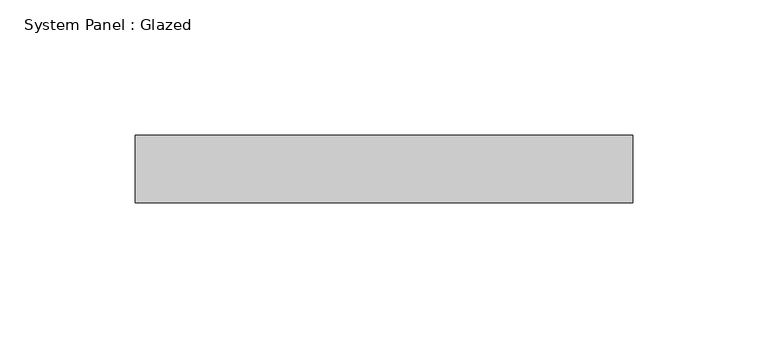
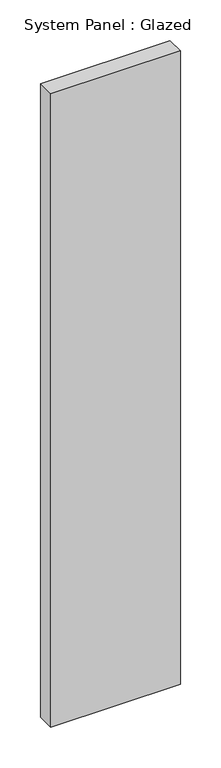
"""IFC4 building model written with IfcOpenShell, lengths in millimetres: plate geometry, System Panel : Glazed."""

import ifcopenshell
import ifcopenshell.guid

model = None  # the IFC model being written
_history = None  # IfcOwnerHistory: only IFC2X3 demands one
_inside = {}  # id of a spatial element -> (the spatial element, [elements in it])
_under = {}  # id of a project, library or spatial element -> (it, [spatial elements below it])
_declared = {}  # id of a project -> (the project, [libraries it declares])
_typed = {}  # id of a type object -> (the type object, [elements of that type])
_made_of = {}  # id of a material, layer set ... -> (it, [elements and type objects made of it])


def new_model(schema):
    """Start an empty IFC model of exactly this schema.

    Asked for "IFC4X3", IfcOpenShell would pick the latest addendum, in which some entities
    have other attributes; the version numbers below select the first issue.
    IFC2X3 requires an IfcOwnerHistory on every rooted entity: one is made here for all.
    """
    global model, _history
    if schema == "IFC4X3":
        model = ifcopenshell.file(schema_version=(4, 3, 0, 0))
    else:
        model = ifcopenshell.file(schema=schema)
    _inside.clear()
    _under.clear()
    _declared.clear()
    _typed.clear()
    _made_of.clear()
    _history = None
    if model.schema == "IFC2X3":
        org = make("IfcOrganization", Name="unknown")
        user = make(
            "IfcPersonAndOrganization",
            ThePerson=make("IfcPerson", FamilyName="unknown"),
            TheOrganization=org,
        )
        app = make(
            "IfcApplication",
            ApplicationDeveloper=org,
            Version="unknown",
            ApplicationFullName="unknown",
            ApplicationIdentifier="unknown",
        )
        _history = make(
            "IfcOwnerHistory",
            OwningUser=user,
            OwningApplication=app,
            ChangeAction="ADDED",
            CreationDate=0,
        )
    return model


def make(cls, **values):
    """One entity of the class cls with the attributes given. An attribute that is None is left unset."""
    return model.create_entity(
        cls, **{name: value for name, value in values.items() if value is not None}
    )


def rooted(cls, **values):
    """An entity with a GlobalId (a new one), such as an element, a storey or a relation."""
    return make(cls, GlobalId=ifcopenshell.guid.new(), OwnerHistory=_history, **values)


def si_unit(unit_type, name, prefix=None):
    """IfcSIUnit, for example si_unit("LENGTHUNIT", "METRE", prefix="MILLI")."""
    return make("IfcSIUnit", UnitType=unit_type, Prefix=prefix, Name=name)


def assignment(units):
    """IfcUnitAssignment: the units of a project."""
    return None if units is None else make("IfcUnitAssignment", Units=units)


def point(xyz):
    """IfcCartesianPoint."""
    return None if xyz is None else make("IfcCartesianPoint", Coordinates=xyz)


def direction(xyz):
    """IfcDirection."""
    return None if xyz is None else make("IfcDirection", DirectionRatios=xyz)


def frame(location, z_axis=None, x_axis=None):
    """IfcAxis2Placement3D, a coordinate frame: its origin and axes. An axis left out is left unset."""
    return make(
        "IfcAxis2Placement3D",
        Location=point(location),
        Axis=direction(z_axis),
        RefDirection=direction(x_axis),
    )


def origin():
    """The frame at (0, 0, 0) with its axes left unset."""
    return frame((0.0, 0.0, 0.0))


def origin_with_axes():
    """The frame at (0, 0, 0) with the z axis (0, 0, 1) and the x axis (1, 0, 0) written out."""
    return frame((0.0, 0.0, 0.0), z_axis=(0.0, 0.0, 1.0), x_axis=(1.0, 0.0, 0.0))


def place(relative_to, where):
    """IfcLocalPlacement: puts the frame where relative to a parent placement (None: the world)."""
    return make(
        "IfcLocalPlacement", PlacementRelTo=relative_to, RelativePlacement=where
    )


def context(
    kind, dimensions, precision=None, world=None, true_north=None, identifier=None
):
    """IfcGeometricRepresentationContext, for example the 3D "Model" context."""
    return make(
        "IfcGeometricRepresentationContext",
        ContextIdentifier=identifier,
        ContextType=kind,
        CoordinateSpaceDimension=dimensions,
        Precision=precision,
        WorldCoordinateSystem=world,
        TrueNorth=true_north,
    )


def project(units=None, contexts=None):
    """IfcProject with its units and contexts."""
    return rooted(
        "IfcProject",
        Name="project",
        RepresentationContexts=contexts,
        UnitsInContext=assignment(units),
    )


def spatial(cls, under=None, at=None, **own):
    """A site, building, storey or space (cls), placed at a placement, below another one or the project."""
    s = rooted(cls, ObjectPlacement=at, **own)
    if under is not None:
        _under.setdefault(under.id(), (under, []))[1].append(s)
    return s


def polyline(points):
    """IfcPolyline through the points."""
    return make("IfcPolyline", Points=[point(p) for p in points])


def outline(outer, holes=None, kind="AREA"):
    """IfcArbitraryClosedProfileDef: a profile drawn as a closed curve; with holes, ...WithVoids."""
    if holes is None:
        return make("IfcArbitraryClosedProfileDef", ProfileType=kind, OuterCurve=outer)
    return make(
        "IfcArbitraryProfileDefWithVoids",
        ProfileType=kind,
        OuterCurve=outer,
        InnerCurves=holes,
    )


def extrude(swept, where, along, depth):
    """IfcExtrudedAreaSolid: the profile swept, set in the frame where, extruded along a direction by depth."""
    return make(
        "IfcExtrudedAreaSolid",
        SweptArea=swept,
        Position=where,
        ExtrudedDirection=direction(along),
        Depth=depth,
    )


def shape(context_of_items, identifier, shape_type, items):
    """IfcShapeRepresentation: the items that make up one representation, for example the "Body"."""
    return make(
        "IfcShapeRepresentation",
        ContextOfItems=context_of_items,
        RepresentationIdentifier=identifier,
        RepresentationType=shape_type,
        Items=items,
    )


def source(mapping_origin, context_of_items, identifier, shape_type, items):
    """IfcRepresentationMap: a shape defined once, which mapped items show again and again."""
    return make(
        "IfcRepresentationMap",
        MappingOrigin=mapping_origin,
        MappedRepresentation=shape(context_of_items, identifier, shape_type, items),
    )


def transform(
    local_origin,
    x_axis=None,
    y_axis=None,
    z_axis=None,
    scale=None,
    scale2=None,
    scale3=None,
    uniform=True,
):
    """IfcCartesianTransformationOperator3D, or its non-uniform kind. x_axis, y_axis, z_axis: its Axis1, 2, 3."""
    if uniform:
        return make(
            "IfcCartesianTransformationOperator3D",
            Axis1=direction(x_axis),
            Axis2=direction(y_axis),
            LocalOrigin=point(local_origin),
            Scale=scale,
            Axis3=direction(z_axis),
        )
    return make(
        "IfcCartesianTransformationOperator3DnonUniform",
        Axis1=direction(x_axis),
        Axis2=direction(y_axis),
        LocalOrigin=point(local_origin),
        Scale=scale,
        Axis3=direction(z_axis),
        Scale2=scale2,
        Scale3=scale3,
    )


def mapped(mapping_source, mapping_target):
    """IfcMappedItem: shows the shape of a source again, moved by a transform."""
    return make(
        "IfcMappedItem", MappingSource=mapping_source, MappingTarget=mapping_target
    )


def made_of(thing, what):
    """Note that an element or type object is made of a material, layer set ...; save() writes the relation."""
    if what is not None:
        _made_of.setdefault(what.id(), (what, []))[1].append(thing)
    return thing


def element(
    cls,
    number,
    at=None,
    inside=None,
    cuts=None,
    type_object=None,
    material=None,
    context=None,
    identifier="Body",
    shape_type=None,
    held_by="IfcProductDefinitionShape",
    body=None,
    shapes=None,
    **own,
):
    """One element of the class cls, such as IfcWall. Its Tag is "e" and its number.

    at: its placement. inside: the storey or other place that contains it. cuts: it is an
    opening in that element (IfcRelVoidsElement). A single representation is given by context,
    identifier, shape_type and body (its items); several are given by shapes. held_by: the class
    of the entity that holds the representations. save() writes the other relations.
    """
    e = rooted(cls, Tag="e%d" % number, ObjectPlacement=at, **own)
    if body is not None:
        shapes = [shape(context, identifier, shape_type, body)]
    if shapes is not None:
        e.Representation = make(held_by, Representations=shapes)
    if inside is not None:
        _inside.setdefault(inside.id(), (inside, []))[1].append(e)
    if cuts is not None:
        rooted(
            "IfcRelVoidsElement", RelatingBuildingElement=cuts, RelatedOpeningElement=e
        )
    if type_object is not None:
        _typed.setdefault(type_object.id(), (type_object, []))[1].append(e)
    return made_of(e, material)


def aggregate(whole, parts):
    """IfcRelAggregates: a whole, such as a stair, and the parts it consists of."""
    return rooted("IfcRelAggregates", RelatingObject=whole, RelatedObjects=parts)


def save(model, path):
    """Write the relations noted so far, then the file.

    IfcRelAggregates (storeys below a building ...), IfcRelContainedInSpatialStructure (elements
    in a storey), IfcRelDefinesByType, IfcRelAssociatesMaterial and IfcRelDeclares: one each for
    every whole, place, type object, material and project.
    """
    for whole, parts in _under.values():
        aggregate(whole, parts)
    for where, things in _inside.values():
        rooted(
            "IfcRelContainedInSpatialStructure",
            RelatedElements=things,
            RelatingStructure=where,
        )
    for kind, things in _typed.values():
        rooted("IfcRelDefinesByType", RelatedObjects=things, RelatingType=kind)
    for what, things in _made_of.values():
        rooted("IfcRelAssociatesMaterial", RelatedObjects=things, RelatingMaterial=what)
    for by, libraries in _declared.values():
        rooted("IfcRelDeclares", RelatingContext=by, RelatedDefinitions=libraries)
    model.write(path)


def system_panel_glazed_af8baef6(model_context):
    return source(origin(), model_context, "Body", "SweptSolid", [
        extrude(outline(polyline([(91.9191919, 24.5), (-91.9191919, 24.5), (-91.9191919, 49.5), (91.9191919, 49.5), (91.9191919, 24.5)])), origin_with_axes(), (0.0, 0.0, 1.0), 950.0),
    ])


if __name__ == "__main__":
    model = new_model("IFC4")
    model_context = context("Model", 3, world=origin())
    ifc_project = project(units=[si_unit("LENGTHUNIT", "METRE", prefix="MILLI")], contexts=[model_context])
    site = spatial("IfcSite", under=ifc_project)
    building = spatial("IfcBuilding", under=site)
    placement = place(None, origin())
    system_panel_glazed_shape = system_panel_glazed_af8baef6(model_context)
    element("IfcPlate", 1, ObjectType="System Panel : Glazed", at=placement, inside=building, context=model_context, shape_type="MappedRepresentation", body=[
        mapped(system_panel_glazed_shape, transform((0.0, 0.0, 0.0), x_axis=(1.0, 0.0, 0.0), y_axis=(0.0, 1.0, 0.0), z_axis=(0.0, 0.0, 1.0))),
    ])
    save(model, "model.ifc")

# Revit data of these elements
# Element 1 (IfcPlate, "System Panel : Glazed")
#   Materials on its faces: "Glass"
# Materials
#   "Glass": class "Glass", colour RGB 218 227 224, transparency 0.85, Description = "Soda Lime Glass", Cost = 0
